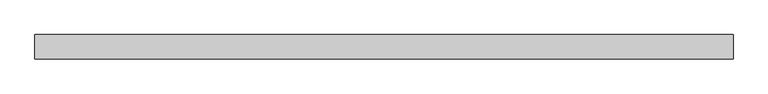
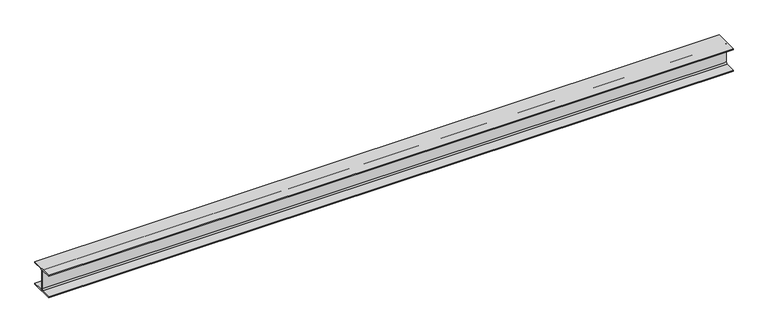
"""IFC4 building model written with IfcOpenShell, lengths in millimetres: beam geometry, 0912_Steel Framing_H-KSD3502 : H_SB_ASB_H-300x300x10x15."""

from ifc_helpers import new_model, si_unit, point, frame, frame_2d, origin, place, context, project, spatial, polyline, circle_curve, trimmed, segment, composite_curve, outline, extrude, source, transform, mapped, element, save


def beam_ce788f5f(model_context):
    return source(origin(), model_context, "Body", "SweptSolid", [
        extrude(outline(composite_curve([segment(polyline([(-150.0, -135.0), (-23.0, -135.0)]), True, "CONTINUOUS"), segment(trimmed(circle_curve(frame_2d((-23.0, -117.0)), 18.0), [point((-23.0, -135.0))], [point((-5.0, -117.0))], True, "CARTESIAN"), True, "CONTINUOUS"), segment(polyline([(-5.0, -117.0), (-5.0, 117.0)]), True, "CONTINUOUS"), segment(trimmed(circle_curve(frame_2d((-23.0, 117.0)), 18.0), [point((-5.0, 117.0))], [point((-23.0, 135.0))], True, "CARTESIAN"), True, "CONTINUOUS"), segment(polyline([(-23.0, 135.0), (-150.0, 135.0), (-150.0, 150.0), (150.0, 150.0), (150.0, 135.0), (23.0, 135.0)]), True, "CONTINUOUS"), segment(trimmed(circle_curve(frame_2d((23.0, 117.0)), 18.0), [point((23.0, 135.0))], [point((5.0, 117.0))], True, "CARTESIAN"), True, "CONTINUOUS"), segment(polyline([(5.0, 117.0), (5.0, -117.0)]), True, "CONTINUOUS"), segment(trimmed(circle_curve(frame_2d((23.0, -117.0)), 18.0), [point((5.0, -117.0))], [point((23.0, -135.0))], True, "CARTESIAN"), True, "CONTINUOUS"), segment(polyline([(23.0, -135.0), (150.0, -135.0), (150.0, -150.0), (-150.0, -150.0), (-150.0, -135.0)]), True, "CONTINUOUS")], self_intersect=False)), frame((-4331.4958952, 0.0, 0.0), z_axis=(1.0, 0.0, 0.0), x_axis=(0.0, 1.0, 0.0)), (0.0, 0.0, 1.0), 8594.5528849),
    ])


if __name__ == "__main__":
    model = new_model("IFC4")
    model_context = context("Model", 3, world=origin())
    ifc_project = project(units=[si_unit("LENGTHUNIT", "METRE", prefix="MILLI")], contexts=[model_context])
    site = spatial("IfcSite", under=ifc_project)
    building = spatial("IfcBuilding", under=site)
    placement = place(None, origin())
    beam_shape = beam_ce788f5f(model_context)
    element("IfcBeam", 1, ObjectType="0912_Steel Framing_H-KSD3502 : H_SB_ASB_H-300x300x10x15", at=placement, inside=building, context=model_context, shape_type="MappedRepresentation", body=[
        mapped(beam_shape, transform((0.0, 0.0, 0.0), x_axis=(1.0, 0.0, 0.0), y_axis=(0.0, 1.0, 0.0), z_axis=(0.0, 0.0, 1.0))),
    ])
    save(model, "model.ifc")

# Revit data of these elements
# Type "0912_Steel Framing_H-KSD3502 : H_SB_ASB_H-300x300x10x15"
#   H_WM Code_1 = "S01AA001-00001 | Main Steel Structure Fabrication Work | Shelter/Building | Heavy Steel - Standard (Weight≥90KG/M) | Material: (   )"
#   H_WM Code_2 = "S03AA027-00001 | Main Steel Structure Erection Work | Shelter/Building | Heavy Steel (Weight≥90KG/M) | Material: (   )"
#   H_WM Code_3 = "S01AA010-00001 | Main Steel Structure Fabrication Work | Shelter/Building | Steel Painting/Coating | for Non-Fireproofed Steel Surface, Surface Preparation, Primer, Second & Final Coat | Material: (   )"
#   H_Q'ty Cal Type Tag = "SB-Q2"
#   Width = 30.0 cm
#   Web Thickness = 1.0 cm
#   Web Fillet = 1.8 cm
#   Warping Constant = 1370000.0 cm⁶
#   W = 0
#   Torsional Moment of Inertia = 77.00 cm⁴
#   Section Area = 119.8 cm²
#   Plastic Modulus weak axis = 684.0 cm³
#   Plastic Modulus strong axis = 1500.0 cm³
#   Perimeter = 1.75 m²/m
#   Nominal Weight = 94.00 kgf/m
#   Moment of Inertia weak axis = 6750.00 cm⁴
#   Moment of Inertia strong axis = 20400.00 cm⁴
#   Height = 30.0 cm
#   Flange Thickness = 1.5 cm
#   Elastic Modulus weak axis = 450.0 cm³
#   Elastic Modulus strong axis = 1360.0 cm³
#   Centroid Vertical = 15.0 cm
#   Centroid Horizontal = 15.0 cm
#   Ix = 204000000
#   Length [instance default] = 1.5240 m
#   Zx = 1500000
#   b = 0.3000 m
#   h = 0.3000 m
#   r = 0.0180 m
#   s = 0.0100 m
#   t = 0.0150 m
#   A = 0.01198 m²
#   Structural Material [instance default] = Steel, 45-345
#   Assembly Code = ""
# Element 1 (IfcBeam, "0912_Steel Framing_H-KSD3502 : H_SB_ASB_H-300x300x10x15")
#   Structural Material = none
# Materials
#   "Steel, 45-345": class "Metal", colour RGB 189 187 185, transparency 0, Description = "Steel 345 MPa", Cost = 0
